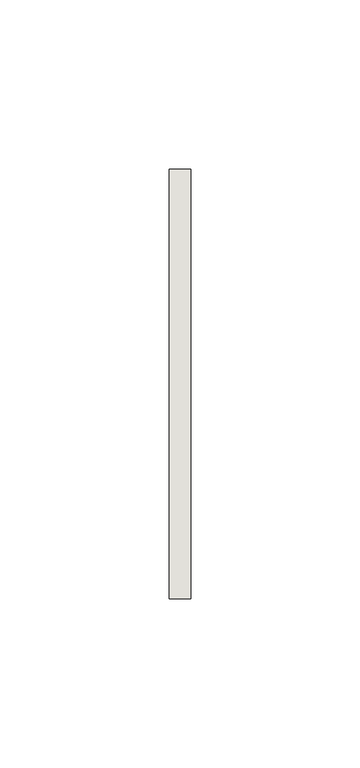
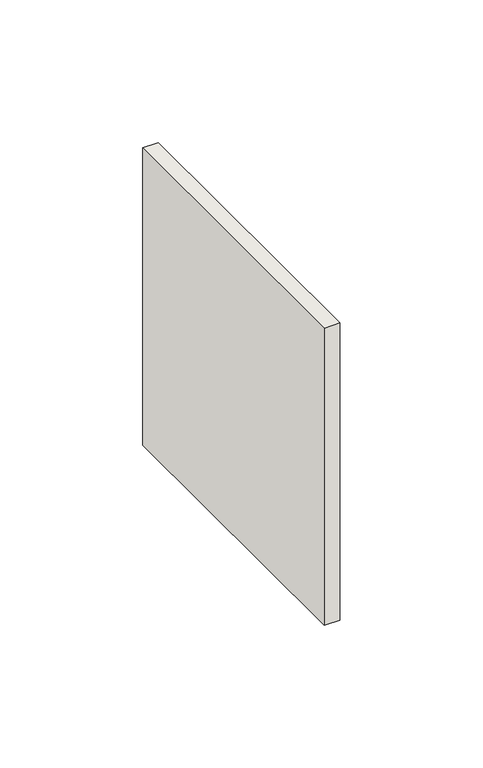
"""IFC4 building model written with IfcOpenShell, lengths in millimetres: wall geometry, TURNBUCKLET PLATE4 : TURNBUCKLET PLATE."""

import ifcopenshell
import ifcopenshell.guid

model = None  # the IFC model being written
_history = None  # IfcOwnerHistory: only IFC2X3 demands one
_inside = {}  # id of a spatial element -> (the spatial element, [elements in it])
_under = {}  # id of a project, library or spatial element -> (it, [spatial elements below it])
_declared = {}  # id of a project -> (the project, [libraries it declares])
_typed = {}  # id of a type object -> (the type object, [elements of that type])
_made_of = {}  # id of a material, layer set ... -> (it, [elements and type objects made of it])


def new_model(schema):
    """Start an empty IFC model of exactly this schema.

    Asked for "IFC4X3", IfcOpenShell would pick the latest addendum, in which some entities
    have other attributes; the version numbers below select the first issue.
    IFC2X3 requires an IfcOwnerHistory on every rooted entity: one is made here for all.
    """
    global model, _history
    if schema == "IFC4X3":
        model = ifcopenshell.file(schema_version=(4, 3, 0, 0))
    else:
        model = ifcopenshell.file(schema=schema)
    _inside.clear()
    _under.clear()
    _declared.clear()
    _typed.clear()
    _made_of.clear()
    _history = None
    if model.schema == "IFC2X3":
        org = make("IfcOrganization", Name="unknown")
        user = make(
            "IfcPersonAndOrganization",
            ThePerson=make("IfcPerson", FamilyName="unknown"),
            TheOrganization=org,
        )
        app = make(
            "IfcApplication",
            ApplicationDeveloper=org,
            Version="unknown",
            ApplicationFullName="unknown",
            ApplicationIdentifier="unknown",
        )
        _history = make(
            "IfcOwnerHistory",
            OwningUser=user,
            OwningApplication=app,
            ChangeAction="ADDED",
            CreationDate=0,
        )
    return model


def make(cls, **values):
    """One entity of the class cls with the attributes given. An attribute that is None is left unset."""
    return model.create_entity(
        cls, **{name: value for name, value in values.items() if value is not None}
    )


def rooted(cls, **values):
    """An entity with a GlobalId (a new one), such as an element, a storey or a relation."""
    return make(cls, GlobalId=ifcopenshell.guid.new(), OwnerHistory=_history, **values)


def si_unit(unit_type, name, prefix=None):
    """IfcSIUnit, for example si_unit("LENGTHUNIT", "METRE", prefix="MILLI")."""
    return make("IfcSIUnit", UnitType=unit_type, Prefix=prefix, Name=name)


def assignment(units):
    """IfcUnitAssignment: the units of a project."""
    return None if units is None else make("IfcUnitAssignment", Units=units)


def point(xyz):
    """IfcCartesianPoint."""
    return None if xyz is None else make("IfcCartesianPoint", Coordinates=xyz)


def direction(xyz):
    """IfcDirection."""
    return None if xyz is None else make("IfcDirection", DirectionRatios=xyz)


def frame(location, z_axis=None, x_axis=None):
    """IfcAxis2Placement3D, a coordinate frame: its origin and axes. An axis left out is left unset."""
    return make(
        "IfcAxis2Placement3D",
        Location=point(location),
        Axis=direction(z_axis),
        RefDirection=direction(x_axis),
    )


def origin():
    """The frame at (0, 0, 0) with its axes left unset."""
    return frame((0.0, 0.0, 0.0))


def place(relative_to, where):
    """IfcLocalPlacement: puts the frame where relative to a parent placement (None: the world)."""
    return make(
        "IfcLocalPlacement", PlacementRelTo=relative_to, RelativePlacement=where
    )


def context(
    kind, dimensions, precision=None, world=None, true_north=None, identifier=None
):
    """IfcGeometricRepresentationContext, for example the 3D "Model" context."""
    return make(
        "IfcGeometricRepresentationContext",
        ContextIdentifier=identifier,
        ContextType=kind,
        CoordinateSpaceDimension=dimensions,
        Precision=precision,
        WorldCoordinateSystem=world,
        TrueNorth=true_north,
    )


def project(units=None, contexts=None):
    """IfcProject with its units and contexts."""
    return rooted(
        "IfcProject",
        Name="project",
        RepresentationContexts=contexts,
        UnitsInContext=assignment(units),
    )


def spatial(cls, under=None, at=None, **own):
    """A site, building, storey or space (cls), placed at a placement, below another one or the project."""
    s = rooted(cls, ObjectPlacement=at, **own)
    if under is not None:
        _under.setdefault(under.id(), (under, []))[1].append(s)
    return s


def polyline(points):
    """IfcPolyline through the points."""
    return make("IfcPolyline", Points=[point(p) for p in points])


def outline(outer, holes=None, kind="AREA"):
    """IfcArbitraryClosedProfileDef: a profile drawn as a closed curve; with holes, ...WithVoids."""
    if holes is None:
        return make("IfcArbitraryClosedProfileDef", ProfileType=kind, OuterCurve=outer)
    return make(
        "IfcArbitraryProfileDefWithVoids",
        ProfileType=kind,
        OuterCurve=outer,
        InnerCurves=holes,
    )


def extrude(swept, where, along, depth):
    """IfcExtrudedAreaSolid: the profile swept, set in the frame where, extruded along a direction by depth."""
    return make(
        "IfcExtrudedAreaSolid",
        SweptArea=swept,
        Position=where,
        ExtrudedDirection=direction(along),
        Depth=depth,
    )


def shape(context_of_items, identifier, shape_type, items):
    """IfcShapeRepresentation: the items that make up one representation, for example the "Body"."""
    return make(
        "IfcShapeRepresentation",
        ContextOfItems=context_of_items,
        RepresentationIdentifier=identifier,
        RepresentationType=shape_type,
        Items=items,
    )


def source(mapping_origin, context_of_items, identifier, shape_type, items):
    """IfcRepresentationMap: a shape defined once, which mapped items show again and again."""
    return make(
        "IfcRepresentationMap",
        MappingOrigin=mapping_origin,
        MappedRepresentation=shape(context_of_items, identifier, shape_type, items),
    )


def transform(
    local_origin,
    x_axis=None,
    y_axis=None,
    z_axis=None,
    scale=None,
    scale2=None,
    scale3=None,
    uniform=True,
):
    """IfcCartesianTransformationOperator3D, or its non-uniform kind. x_axis, y_axis, z_axis: its Axis1, 2, 3."""
    if uniform:
        return make(
            "IfcCartesianTransformationOperator3D",
            Axis1=direction(x_axis),
            Axis2=direction(y_axis),
            LocalOrigin=point(local_origin),
            Scale=scale,
            Axis3=direction(z_axis),
        )
    return make(
        "IfcCartesianTransformationOperator3DnonUniform",
        Axis1=direction(x_axis),
        Axis2=direction(y_axis),
        LocalOrigin=point(local_origin),
        Scale=scale,
        Axis3=direction(z_axis),
        Scale2=scale2,
        Scale3=scale3,
    )


def mapped(mapping_source, mapping_target):
    """IfcMappedItem: shows the shape of a source again, moved by a transform."""
    return make(
        "IfcMappedItem", MappingSource=mapping_source, MappingTarget=mapping_target
    )


def made_of(thing, what):
    """Note that an element or type object is made of a material, layer set ...; save() writes the relation."""
    if what is not None:
        _made_of.setdefault(what.id(), (what, []))[1].append(thing)
    return thing


def element(
    cls,
    number,
    at=None,
    inside=None,
    cuts=None,
    type_object=None,
    material=None,
    context=None,
    identifier="Body",
    shape_type=None,
    held_by="IfcProductDefinitionShape",
    body=None,
    shapes=None,
    **own,
):
    """One element of the class cls, such as IfcWall. Its Tag is "e" and its number.

    at: its placement. inside: the storey or other place that contains it. cuts: it is an
    opening in that element (IfcRelVoidsElement). A single representation is given by context,
    identifier, shape_type and body (its items); several are given by shapes. held_by: the class
    of the entity that holds the representations. save() writes the other relations.
    """
    e = rooted(cls, Tag="e%d" % number, ObjectPlacement=at, **own)
    if body is not None:
        shapes = [shape(context, identifier, shape_type, body)]
    if shapes is not None:
        e.Representation = make(held_by, Representations=shapes)
    if inside is not None:
        _inside.setdefault(inside.id(), (inside, []))[1].append(e)
    if cuts is not None:
        rooted(
            "IfcRelVoidsElement", RelatingBuildingElement=cuts, RelatedOpeningElement=e
        )
    if type_object is not None:
        _typed.setdefault(type_object.id(), (type_object, []))[1].append(e)
    return made_of(e, material)


def aggregate(whole, parts):
    """IfcRelAggregates: a whole, such as a stair, and the parts it consists of."""
    return rooted("IfcRelAggregates", RelatingObject=whole, RelatedObjects=parts)


def save(model, path):
    """Write the relations noted so far, then the file.

    IfcRelAggregates (storeys below a building ...), IfcRelContainedInSpatialStructure (elements
    in a storey), IfcRelDefinesByType, IfcRelAssociatesMaterial and IfcRelDeclares: one each for
    every whole, place, type object, material and project.
    """
    for whole, parts in _under.values():
        aggregate(whole, parts)
    for where, things in _inside.values():
        rooted(
            "IfcRelContainedInSpatialStructure",
            RelatedElements=things,
            RelatingStructure=where,
        )
    for kind, things in _typed.values():
        rooted("IfcRelDefinesByType", RelatedObjects=things, RelatingType=kind)
    for what, things in _made_of.values():
        rooted("IfcRelAssociatesMaterial", RelatedObjects=things, RelatingMaterial=what)
    for by, libraries in _declared.values():
        rooted("IfcRelDeclares", RelatingContext=by, RelatedDefinitions=libraries)
    model.write(path)


def wall_70ac90b7(model_context):
    return source(origin(), model_context, "Body", "SweptSolid", [
        extrude(outline(polyline([(22994.1370052, -1109.9884634), (22994.1370052, -982.9884634), (23000.4870052, -982.9884634), (23000.4870052, -1109.9884634), (22994.1370052, -1109.9884634)])), frame((0.0, 0.0, 4845.2706466), z_axis=(0.0, 0.0, 1.0), x_axis=(1.0, 0.0, 0.0)), (0.0, 0.0, 1.0), 127.0),
    ])


if __name__ == "__main__":
    model = new_model("IFC4")
    model_context = context("Model", 3, world=origin())
    ifc_project = project(units=[si_unit("LENGTHUNIT", "METRE", prefix="MILLI")], contexts=[model_context])
    site = spatial("IfcSite", under=ifc_project)
    building = spatial("IfcBuilding", under=site)
    placement = place(None, origin())
    wall_shape = wall_70ac90b7(model_context)
    element("IfcWall", 1, ObjectType="TURNBUCKLET PLATE4 : TURNBUCKLET PLATE", at=placement, inside=building, context=model_context, shape_type="MappedRepresentation", body=[
        mapped(wall_shape, transform((0.0, 0.0, 0.0), x_axis=(1.0, 0.0, 0.0), y_axis=(0.0, 1.0, 0.0), z_axis=(0.0, 0.0, 1.0))),
    ])
    save(model, "model.ifc")

# Revit data of these elements
# Element 1 (IfcWall, "TURNBUCKLET PLATE4 : TURNBUCKLET PLATE")
#   Materials on its faces: "1/4\" STEEL GUSSET PLATE - (RAW STEEL)"
# Materials
#   "1/4\" STEEL GUSSET PLATE - (RAW STEEL)": class "Metal", colour RGB 189 187 185, transparency 0, Description = "Structural steel 50ksi", Cost = 0
